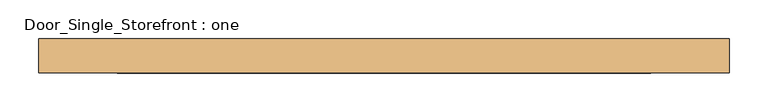
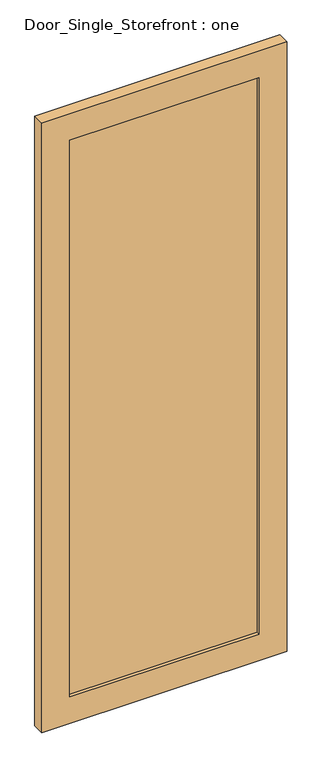
"""IFC4 building model written with IfcOpenShell, lengths in millimetres: door geometry, Door_Single_Storefront : one."""

from ifc_helpers import new_model, si_unit, frame, origin, place, context, project, spatial, polyline, outline, extrude, source, transform, mapped, element, save


def door_single_storefront_one_82dfc470(model_context):
    return source(origin(), model_context, "Body", "SweptSolid", [
        extrude(outline(polyline([(2349.5, -446.88125), (0.0, -446.88125), (0.0, 446.88125), (2349.5, 446.88125), (2349.5, -446.88125)]), holes=[polyline([(101.6, 345.28125), (101.6, -345.28125), (2247.9, -345.28125), (2247.9, 345.28125), (101.6, 345.28125)])]), frame((0.0, 6.35, 0.0), z_axis=(0.0, 1.0, 0.0), x_axis=(0.0, 0.0, 1.0)), (0.0, 0.0, 1.0), 44.45),
        extrude(outline(polyline([(345.28125, 19.05), (-345.28125, 19.05), (-345.28125, 38.1), (345.28125, 38.1), (345.28125, 19.05)])), frame((0.0, 0.0, 101.6), z_axis=(0.0, 0.0, 1.0), x_axis=(1.0, 0.0, 0.0)), (0.0, 0.0, 1.0), 2146.3),
    ])


if __name__ == "__main__":
    model = new_model("IFC4")
    model_context = context("Model", 3, world=origin())
    ifc_project = project(units=[si_unit("LENGTHUNIT", "METRE", prefix="MILLI")], contexts=[model_context])
    site = spatial("IfcSite", under=ifc_project)
    building = spatial("IfcBuilding", under=site)
    placement = place(None, origin())
    door_single_storefront_one_shape = door_single_storefront_one_82dfc470(model_context)
    element("IfcDoor", 1, ObjectType="Door_Single_Storefront : one", at=placement, inside=building, context=model_context, shape_type="MappedRepresentation", body=[
        mapped(door_single_storefront_one_shape, transform((0.0, 0.0, 0.0), x_axis=(1.0, 0.0, 0.0), y_axis=(0.0, 1.0, 0.0), z_axis=(0.0, 0.0, 1.0))),
    ])
    save(model, "model.ifc")

# Revit data of these elements
# Type "Door_Single_Storefront : one"
#   Type Mark = "27"
#   Analytic Construction = "<None>"
#   Stile_Width = 0' - 4"
#   Door_Thickness = 0' - 1 3/4"
#   Door_Offset = 0' - 2"
#   Glass_Material = Glass
#   Frame_Material = Aluminum
#   Function = (empty or 0)
# Element 1 (IfcDoor, "Door_Single_Storefront : one")
#   Materials on its faces: "Aluminum", "Glass"
# Materials
#   "Glass": class "Glass", colour RGB 0 128 192, transparency 0.75, Description = "Soda Lime Glass", Cost = 0
#   "Aluminum": class "Metal", colour RGB 247 247 247, transparency 0, Description = "Aluminum 6061", Cost = 0
